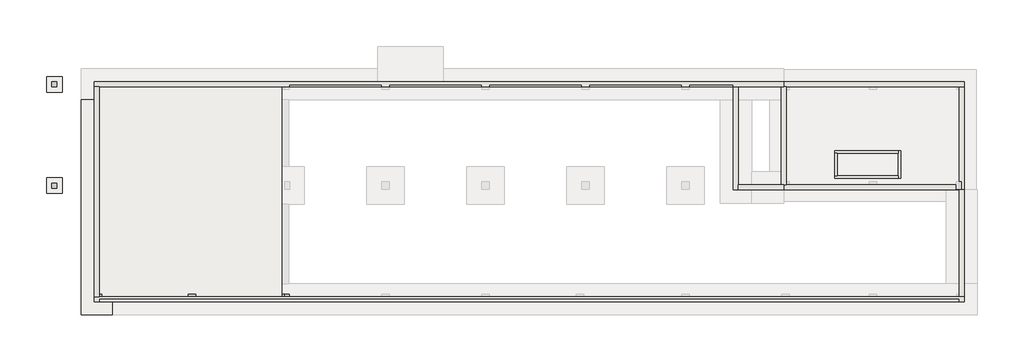
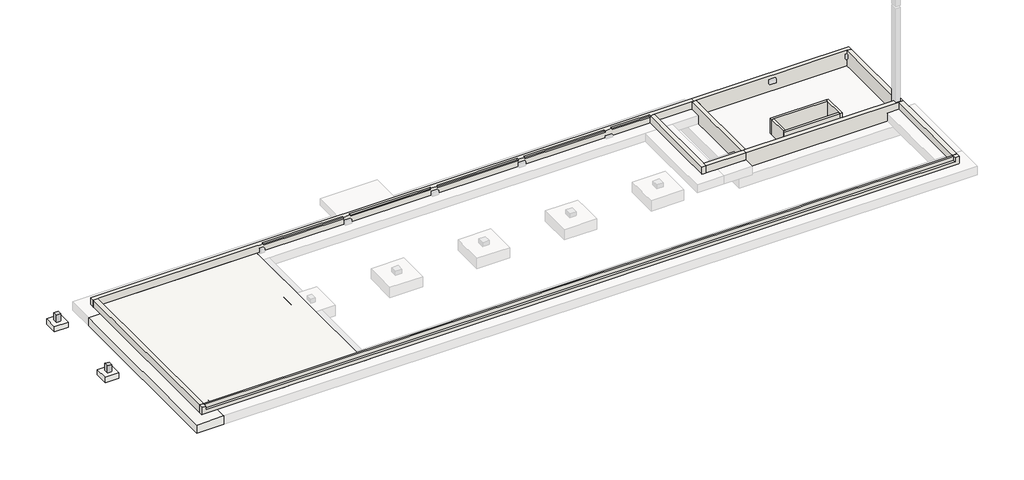
# Not in any storey, part 1 of 2: 14 walls, 5 columns, 3 slabs, 2 beams, 1 footing.
# Revit data of these elements (continued)
# Type "H_SF_AR_B01_Wall FDN_T800" (continued)
#   H_WM Code_6 = "A01ZZ001-00012 |  | M3 | Earth Work | - | Excavation | Soil, Mech. |  | Manual Excavation Above GWL |  |  |  | A01ZZ001-00012 Earth Work - Excavation Soil, Mech.      Manual Excavation Above GWL  | Above GWL"
#   H_WM Code_7 = "A01ZZ001-00013 |  | M3 | Earth Work | - | Excavation | Soil, Mech. |  | Manual Excavation Below GWL |  |  |  | A01ZZ001-00013 Earth Work - Excavation Soil, Mech.      Manual Excavation Below GWL  | Below GWL"
#   H_WM Code_8 = "A01ZZ003-00001 |  | M3 | Earth Work | - | Backfill | Re-use, Soil |  |  |  | Compaction=(  )% |  | A01ZZ003-00001 Earth Work - Backfill Re-use, Soil        | Compaction=( 95 )%"
#   H_WM Code_9 = "A01ZZ004-00001 |  | M3 | Earth Work | - | Disposal | Soil |  |  |  | Disposal Distance=Appx. (  )km from Site |  | A01ZZ004-00001 Earth Work - Disposal Soil        | Disposal Distance=Appx. (20 )km from Site"
#   H_WM Code_10 = "A03AH056-00001 |  | M2 | Concrete Work | Concrete Protective Coating (U/G) | Bitumen/Bituminous/Asphalt Coating |  |  | A03AH056-00001 Concrete Work Concrete Protective Coating (U/G) Bitumen/Bituminous/Asphalt Coating         | *기초바닥 Protection 은 Lean에 적용"
#   H_Rebar ratio = 0.3
# Type "H_FL_AR_S17_RC Slab T150_B1S1"
#   Keynote = ""
#   Type Comments = "CV-AG"
#   Description = ""
#   Type Mark = "B1S1"
#   H_Q'ty Cal Type Tag = "FL-Q1"
#   H_WM Code_1 = "A03AF032-00022 |  | M3 | Concrete Work | Superstructure Work | Structural Concrete | Cement Type-1 | 25MPa ≤ F'c (Cylinder Strength) < 30MPa |  |  |  |  | A03AF032-00022 Concrete Work Superstructure Work Structural Concrete  Cement Type-1 25MPa ≤ F'c (Cylinder Strength) < 30MPa      | ASTM C150 Type I or Type IA \nF'c (Cylinder Strength) = 28MPa"
#   H_WM Code_2 = "A03AF037-00003 |  | TON | Concrete Work | Superstructure Work | Rebar Work | Deformed Bar (Non-Coat.) | 300MPa<Fy≤400MPa |  |  |  |  | A03AF037-00003 Concrete Work Superstructure Work Rebar Work Deformed Bar (Non-Coat.)  300MPa<Fy≤400MPa      | KS D3504 SD400 (Fy=400MPa)"
#   H_WM Code_3 = "A03AF036-00001 |  | M2 | Concrete Work | Superstructure Work | Form Work (1 time in use) | Flat Form | Dressed Lumber, Plywood or Steel Form(Wood Planks are not Allowed) incl. Chamfer |  |  |  | A03AF036-00001 Concrete Work Superstructure Work Form Work (1 time in use) Flat Form     Dressed Lumber, Plywood or Steel Form(Wood Planks are not Allowed) incl. Chamfer   |"
#   H_WM Code_4 = "A04AS173-00001 |  | M2 | Finishing Work | Exterior/Interior Finish Work | Steel Trowel Finish |  |  |  |  | A04AS173-00001 Finishing Work Exterior/Interior Finish Work Steel Trowel Finish         |"
#   H_Rebar ratio = 0.1
#   Function = 1
#   Layers, outside or top first: 150 mm "00_Concrete_Reinf. Conc." (function 1)
# Type "Foundation Rectangular (Non-Pile) : H_SF_AR_S18_W1250xL1250xT500_Bitumen_F2"
#   Type Comments = "UG"
#   Type Mark = "F2"
#   H_Q'ty Cal Type Tag = "SB-Q1"
#   H_WM Code_1 = "A03AF032-00022 |  | M3 | Concrete Work | Superstructure Work | Structural Concrete | Cement Type-1 | 25MPa ≤ F'c (Cylinder Strength) < 30MPa |  |  |  |  | A03AF032-00022 Concrete Work Superstructure Work Structural Concrete  Cement Type-1 25MPa ≤ F'c (Cylinder Strength) < 30MPa      |  F'c (Cylinder Strength) = 24MPa"
#   H_WM Code_2 = "A03AD037-00002 |  | TON | Concrete Work | Substructure Work | Rebar Work | Deformed Bar (Non-Coat.) | 400MPa<Fy≤470MPa |  |  |  |  | A03AD037-00002 Concrete Work Substructure Work Rebar Work Deformed Bar (Non-Coat.)  400MPa<Fy≤470MPa      | ASTM A615 GRADE 60 (Fy=420MPa)"
#   H_WM Code_3 = "A03AF036-00001 |  | M2 | Concrete Work | Superstructure Work | Form Work (1 time in use) | Flat Form | Dressed Lumber, Plywood or Steel Form(Wood Planks are not Allowed) incl. Chamfer |  |  |  | A03AF036-00001 Concrete Work Superstructure Work Form Work (1 time in use) Flat Form     Dressed Lumber, Plywood or Steel Form(Wood Planks are not Allowed) incl. Chamfer   |"
#   Top bar = "D25@300"
#   Description = "UG Shallow Foundation"
#   Bottom bar = "D20@300"
#   Width = 1250 mm
#   Length = 1250 mm
#   Foundation Thickness = 500 mm
#   Structural Material [instance default] = none
#   Assembly Code = ""
# Type "H_WA_AR_B02_Ext Wall_RC T400_UG_Bitumen 2"
#   Type Comments = "CV-UG"
#   Type Mark = "W1A"
#   H_Q'ty Cal Type Tag = "WA-Q1"
#   H_WM Code_1 = "A03AF032-00022 |  | M3 | Concrete Work | Superstructure Work | Structural Concrete | Cement Type-1 | 25MPa ≤ F'c (Cylinder Strength) < 30MPa |  |  |  |  | A03AF032-00022 Concrete Work Superstructure Work Structural Concrete  Cement Type-1 25MPa ≤ F'c (Cylinder Strength) < 30MPa      | ASTM C150 Type I or Type IA \nF'c (Cylinder Strength) = 28MPa"
#   H_WM Code_2 = "A03AD037-00002 |  | TON | Concrete Work | Substructure Work | Rebar Work | Deformed Bar (Non-Coat.) | 400MPa<Fy≤470MPa |  |  |  |  | A03AD037-00002 Concrete Work Substructure Work Rebar Work Deformed Bar (Non-Coat.)  400MPa<Fy≤470MPa      | ASTM A615 GRADE 60 (Fy=420MPa)"
#   H_WM Code_3 = "A03AD036-00001 |  | M2 | Concrete Work | Substructure Work | Form Work (1 time in use) | Flat Form | Dressed Lumber, Plywood or Steel Form(Wood Planks are not Allowed) incl. Chamfer |  |  |  | A03AD036-00001 Concrete Work Substructure Work Form Work (1 time in use) Flat Form     Dressed Lumber, Plywood or Steel Form(Wood Planks are not Allowed) incl. Chamfer   |"
#   H_WM Code_4 = "A04AL076-00008 |  | M2 | Finishing Work | Masonry Work | Insulation | Glass Wool (Fiberglass) | Minimum Density of 50 kg/m3 | 100mm≤THK | THK=(  )mm |  | A04AL076-00008 Finishing Work Masonry Work Insulation Glass Wool (Fiberglass)     Minimum Density of 50 kg/m3  100mm≤THK | inside insulation"
#   H_WM Code_5 = "A04AS177-00004 |  | M2 | Finishing Work | Exterior/Interior Finish Work | Gypsumboard Partition Wall (Fixed Type) | Fire Protective Rating: N/A, 2-Layer Gypsum Boards to One Side | w/o Insulation | Including Supporting Frame(Stud) & Accessories | 1-Layer Gypsumboard THK=9.5mm |  |  | A04AS177-00004 Finishing Work Exterior/Interior Finish Work Gypsumboard Partition Wall (Fixed Type) Fire Protective Rating: N/A, 2-Layer Gypsum Boards to One Side   w/o Insulation  Including Supporting Frame(Stud) & Accessories  1-Layer Gypsumboard THK=9.5mm | gypsum board"
#   H_Rebar ratio = 0.12
#   Layers, outside or top first: 400 mm "00_Concrete_Reinf. Conc." (function 1)
# Type "H_WA_AR_B02_Ext Wall_RC T400_UG_Bitumen_W1A"
#   Type Comments = "CV-UG"
#   Type Mark = "W1A"
#   H_Q'ty Cal Type Tag = "WA-Q1"
#   H_WM Code_1 = "A03AD032-00025 |  | M3 | Concrete Work | Substructure Work | Structural Concrete | Cement Type-1 | 20MPa ≤ F'c (Cylinder Strength) < 25MPa |  |  |  |  | A03AD032-00025 Concrete Work Substructure Work Structural Concrete  Cement Type-1 20MPa ≤ F'c (Cylinder Strength) < 25MPa      | ASTM C150 Type I or Type IA \nF'c (Cylinder Strength) = 24MPa"
#   H_WM Code_2 = "A03AD037-00002 |  | TON | Concrete Work | Substructure Work | Rebar Work | Deformed Bar (Non-Coat.) | 400MPa<Fy≤470MPa |  |  |  |  | A03AD037-00002 Concrete Work Substructure Work Rebar Work Deformed Bar (Non-Coat.)  400MPa<Fy≤470MPa      | ASTM A615 GRADE 60 (Fy=420MPa)"
#   H_WM Code_3 = "A03AD036-00001 |  | M2 | Concrete Work | Substructure Work | Form Work (1 time in use) | Flat Form | Dressed Lumber, Plywood or Steel Form(Wood Planks are not Allowed) incl. Chamfer |  |  |  | A03AD036-00001 Concrete Work Substructure Work Form Work (1 time in use) Flat Form     Dressed Lumber, Plywood or Steel Form(Wood Planks are not Allowed) incl. Chamfer   |"
#   H_Rebar ratio = 0.12
#   Layers, outside or top first: 400 mm "00_Concrete_Reinf. Conc." (function 1)
# Type "H_WA_AR_B02_Int Wall_RC_Trench"
#   Type Comments = "CV-UG"
#   Type Mark = "trench"
#   H_Q'ty Cal Type Tag = "WA-Q1"
#   H_WM Code_1 = "A04AS177-00019 |  | M2 | Finishing Work | Exterior/Interior Finish Work | Gypsumboard Partition Wall (Fixed Type) | Fire Protective Rating: N/A, 2-Layer Gypsum Boards to Both Sides | Glass Wool (Fiberglass) | Including Supporting Frame(Stud) & Accessories | 1-Layer Gypsumboard THK=9.5mm | Insulation THK=(  )mm |  | A04AS177-00019 Finishing Work Exterior/Interior Finish Work Gypsumboard Partition Wall (Fixed Type) Fire Protective Rating: N/A, 2-Layer Gypsum Boards to Both Sides   Glass Wool (Fiberglass)  Including Supporting Frame(Stud) & Accessories  1-Layer Gypsumboard THK=9.5mm |"
#   H_WM Code_2 = "A04AL069-00002 |  | M2 | Finishing Work | Masonry Work | Reinforced Concrete Block | w/ All Reinf.(Lath, Steel Tie, Anchor Bar, Mortar, ETC.), Filler, Sealant, Lintel/Sill for Opening, ETC. | 100mm<THK≤200mm | THK=(  )mm |  | A04AL069-00002 Finishing Work Masonry Work Reinforced Concrete Block      w/ All Reinf.(Lath, Steel Tie, Anchor Bar, Mortar, ETC.), Filler, Sealant, Lintel/Sill for Opening, ETC.  100mm<THK≤200mm | THK=( 150)mm"
#   H_Rebar ratio = 0.12
#   Layers, outside or top first: 200 mm "00_Concrete_Reinf. Conc." (function 1)
# Element 1 (IfcBeam, "RC Beam_Rectangular : H_SB_AR_S16_FG_B500xH700_FB1")
#   Comments = ""
#   hec_material3 = none
#   hec_material2 = none
#   hec_material1 = none
#   Structural Material = 00_Concrete_Reinf. Conc.
#   Phase Created = New Construction
#   Materials on its faces: "00_Concrete_Reinf. Conc."
# Element 2 (IfcBeam, "RC Beam_Rectangular : H_SB_AR_S16_FG_B500xH700_FG1")
#   Comments = ""
#   hec_material3 = none
#   hec_material2 = none
#   hec_material1 = none
#   Structural Material = 00_Concrete_Reinf. Conc.
#   Phase Created = New Construction
#   Materials on its faces: "00_Concrete_Reinf. Conc."
# Elements 3, 4, 5 (IfcColumn, "RC_Column_Rectangular : H_SC_AR_S15_UG_W600xL600_C2")
#   Comments = ""
#   hec_material3 = none
#   hec_material2 = none
#   hec_material1 = none
#   Structural Material = 00_Concrete_Reinf. Conc.
#   Phase Created = New Construction
#   Materials on its faces: "00_Concrete_Reinf. Conc."
# Elements 6, 7 (IfcColumn, "RC_Column_Rectangular : H_SC_AR_S15_UG_W400xL400_C3")
#   Comments = ""
#   hec_material3 = none
#   hec_material2 = none
#   hec_material1 = none
#   Structural Material = 00_Concrete_Reinf. Conc.
#   Phase Created = New Construction
#   Materials on its faces: "00_Concrete_Reinf. Conc."
# Element 8 (IfcFooting, "H_SF_AR_B01_Wall FDN_T800")
#   Comments = ""
#   Phase Created = New Construction
#   Materials on its faces: "00_Concrete_Reinf. Conc."
# Element 9 (IfcSlab, "H_FL_AR_S17_RC Slab T150_B1S1")
#   Comments = ""
#   TMP_Element Name = "SS2"
#   Height Offset From Level = 800 mm
#   built-in parameter 1001954 = 1
#   Phase Created = New Construction
#   Materials on its faces: "00_Concrete_Reinf. Conc."
# Elements 10, 11 (IfcSlab, "Foundation Rectangular (Non-Pile) : H_SF_AR_S18_W1250xL1250xT500_Bitumen_F2")
#   Comments = ""
#   Structural Material = 00_Concrete_Reinf. Conc.
#   Phase Created = New Construction
#   Materials on its faces: "00_Concrete_Reinf. Conc."
# Elements 12, 13, 14, 15, 16, 17 (IfcWall, "H_WA_AR_B02_Ext Wall_RC T400_UG_Bitumen 2")
#   Comments = ""
#   built-in parameter 1001111 = 800 mm
#   Top Offset = 0 mm
#   Base Offset = 800 mm
#   wall height = 700 mm
#   Phase Created = New Construction
#   Base Constraint = BOF
#   Top Constraint = TOC
#   Materials on its faces: "00_Concrete_Reinf. Conc."
# Elements 18, 19, 20, 21 (IfcWall, "H_WA_AR_B02_Ext Wall_RC T400_UG_Bitumen_W1A")
#   Comments = ""
#   Top Offset = 0 mm
#   Base Offset = 0 mm
#   wall height = 1500 mm
#   Phase Created = New Construction
#   Base Constraint = BOF
#   Top Constraint = TOC
#   Materials on its faces: "00_Concrete_Reinf. Conc."
# Elements 22, 23, 24, 25 (IfcWall, "H_WA_AR_B02_Int Wall_RC_Trench")
#   Comments = ""
#   Top Offset = 0 mm
#   Base Offset = 0 mm
#   wall height = 1500 mm
#   Phase Created = New Construction
#   Base Constraint = BOF
#   Top Constraint = TOC
#   Materials on its faces: "00_Concrete_Reinf. Conc."
# Materials
#   "00_Concrete_Reinf. Conc.": class "Concrete", colour RGB 176 176 176, transparency 0, Description = "Reinf. Conc.", Cost = 0, Image = Concrete.Cast-In-Place.Flat.Polished.Grey.jpg
